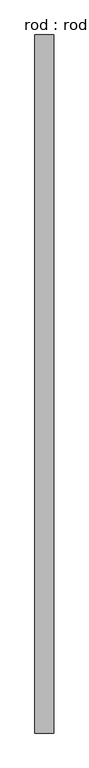
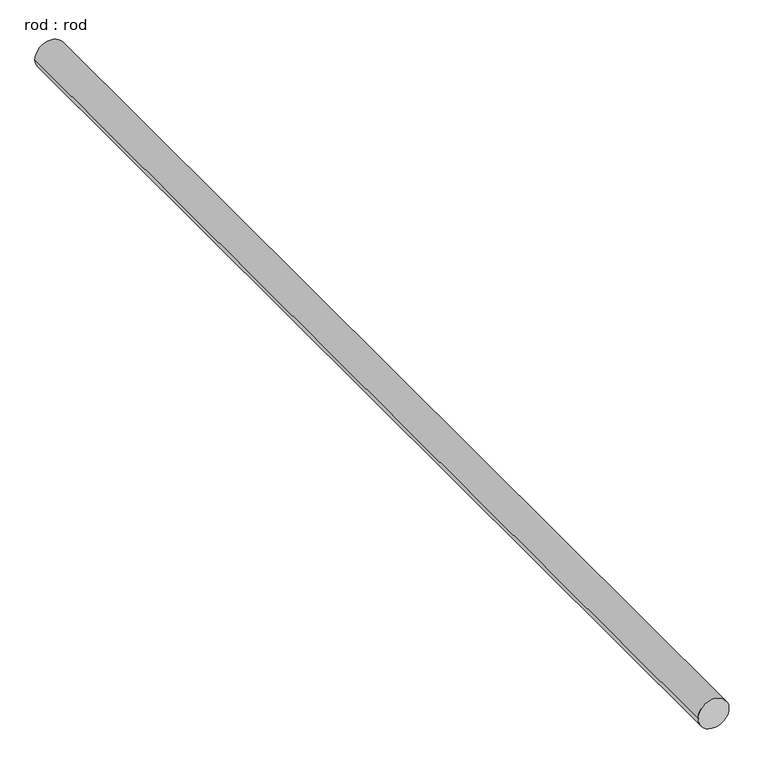
"""IFC4 building model written with IfcOpenShell, lengths in millimetres: proxy geometry, rod : rod."""

from ifc_helpers import new_model, si_unit, point, frame, frame_2d, origin, place, context, project, spatial, circle_curve, trimmed, segment, composite_curve, outline, extrude, source, transform, mapped, element, save


def rod_rod_d696530c(model_context):
    return source(origin(), model_context, "Body", "SweptSolid", [
        extrude(outline(composite_curve([segment(trimmed(circle_curve(frame_2d((0.0108462, 0.0)), 200.0), [point((0.0108462, 200.0))], [point((0.0108462, -200.0))], False, "CARTESIAN"), True, "CONTINUOUS"), segment(trimmed(circle_curve(frame_2d((0.0108462, 0.0)), 200.0), [point((0.0108462, -200.0))], [point((0.0108462, 200.0))], False, "CARTESIAN"), True, "CONTINUOUS")], self_intersect=False)), frame((0.0, -3367.5830404, 0.0), z_axis=(0.0, 1.0, 0.0), x_axis=(0.0, 0.0, 1.0)), (0.0, 0.0, 1.0), 14920.6233114),
    ])


if __name__ == "__main__":
    model = new_model("IFC4")
    model_context = context("Model", 3, world=origin())
    ifc_project = project(units=[si_unit("LENGTHUNIT", "METRE", prefix="MILLI")], contexts=[model_context])
    site = spatial("IfcSite", under=ifc_project)
    building = spatial("IfcBuilding", under=site)
    placement = place(None, origin())
    rod_rod_shape = rod_rod_d696530c(model_context)
    element("IfcBuildingElementProxy", 1, Name="rod : rod", ObjectType="rod : rod", at=placement, inside=building, context=model_context, shape_type="MappedRepresentation", body=[
        mapped(rod_rod_shape, transform((0.0, 0.0, 0.0), x_axis=(1.0, 0.0, 0.0), y_axis=(0.0, 1.0, 0.0), z_axis=(0.0, 0.0, 1.0))),
    ])
    save(model, "model.ifc")

# Revit data of these elements
# Type "rod : rod"
#   Default Elevation = 0
